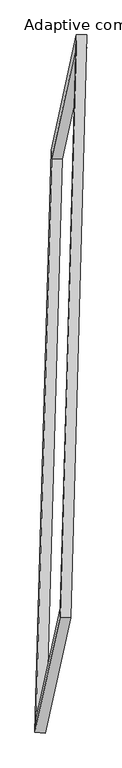
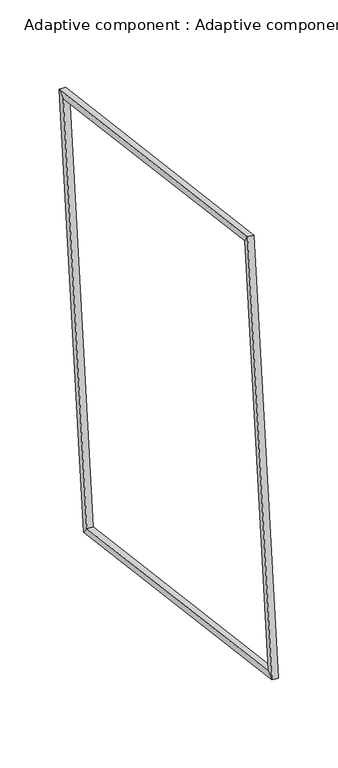
"""IFC4 building model written with IfcOpenShell, lengths in millimetres: proxy geometry, Adaptive component : Adaptive component."""

from ifc_helpers import new_model, si_unit, origin, place, context, project, spatial, faceted_brep, source, transform, mapped, element, save


def adaptive_component_adaptive_component_bb9a7157(model_context):
    return source(origin(), model_context, "Body", "Brep", [
        faceted_brep([(105.7267134, 1725.8142304, 3259.0692176), (170.7489992, 1725.7100933, 3258.5932296), (15.6803984, 1016.8861585, -1149.8866778), (-49.2189784, 1017.5521168, -1145.9164828), (103.4442859, 1651.3300895, 3205.2754611), (-46.9910272, 963.6850729, -1071.4836759), (168.4665717, 1651.2259525, 3204.7994731), (17.9083496, 963.0191146, -1075.4538708), (-84.7538287, -2568.4244863, -569.8844441), (-149.5553169, -2564.2640918, -566.4795504), (-143.735158, -2489.8961606, -512.791549), (-78.9336698, -2494.0565551, -516.1964426), (70.3147721, -1859.6005515, 3838.5954633), (5.3903749, -1856.0019783, 3838.50615), (6.7001551, -1802.2511439, 3763.967588), (71.6245523, -1805.8497172, 3764.0569013)], [[[0, 1, 2, 3]], [[4, 0, 3, 5]], [[6, 4, 5, 7]], [[1, 6, 7, 2]], [[3, 2, 8, 9]], [[5, 3, 9, 10]], [[7, 5, 10, 11]], [[2, 7, 11, 8]], [[9, 8, 12, 13]], [[10, 9, 13, 14]], [[11, 10, 14, 15]], [[8, 11, 15, 12]], [[13, 12, 1, 0]], [[14, 13, 0, 4]], [[15, 14, 4, 6]], [[12, 15, 6, 1]]]),
    ])


if __name__ == "__main__":
    model = new_model("IFC4")
    model_context = context("Model", 3, world=origin())
    ifc_project = project(units=[si_unit("LENGTHUNIT", "METRE", prefix="MILLI")], contexts=[model_context])
    site = spatial("IfcSite", under=ifc_project)
    building = spatial("IfcBuilding", under=site)
    placement = place(None, origin())
    adaptive_component_adaptive_component_shape = adaptive_component_adaptive_component_bb9a7157(model_context)
    element("IfcBuildingElementProxy", 1, Name="Adaptive component : Adaptive component", ObjectType="Adaptive component : Adaptive component", at=placement, inside=building, context=model_context, shape_type="MappedRepresentation", body=[
        mapped(adaptive_component_adaptive_component_shape, transform((0.0, 0.0, 0.0), x_axis=(1.0, 0.0, 0.0), y_axis=(0.0, 1.0, 0.0), z_axis=(0.0, 0.0, 1.0))),
    ])
    save(model, "model.ifc")

# Revit data of these elements
# Type "Adaptive component : Adaptive component"
#   r [instance default] = 2063.125 mm
#   2r [instance default] = 4126.251 mm
#   Number [instance default] = 5
#   Default Elevation = 0
# Element 1 (IfcBuildingElementProxy, "Adaptive component : Adaptive component")
#   r = 2785.576 mm
#   2r = 5571.153 mm
#   Number = 30
